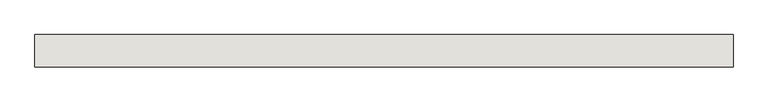
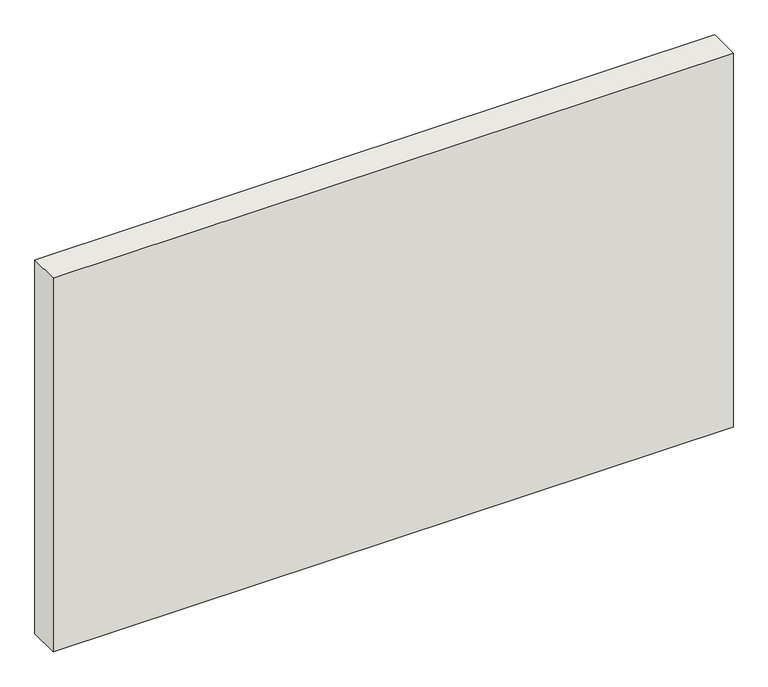
"""IFC4 building model written with IfcOpenShell, lengths in millimetres: wall geometry, Holzwand."""

from ifc_helpers import new_model, si_unit, origin, origin_with_axes, place, context, project, spatial, polyline, outline, extrude, source, transform, mapped, element, save


def wall_2eec8b8f(model_context):
    return source(origin(), model_context, "Body", "SweptSolid", [
        extrude(outline(polyline([(4297.8619019, 200.0), (4297.8619019, 0.0), (0.0, 0.0), (0.0, 200.0), (4297.8619019, 200.0)])), origin_with_axes(), (0.0, 0.0, 1.0), 2500.0),
    ])


if __name__ == "__main__":
    model = new_model("IFC4")
    model_context = context("Model", 3, world=origin())
    ifc_project = project(units=[si_unit("LENGTHUNIT", "METRE", prefix="MILLI")], contexts=[model_context])
    site = spatial("IfcSite", under=ifc_project)
    building = spatial("IfcBuilding", under=site)
    placement = place(None, origin())
    wall_shape = wall_2eec8b8f(model_context)
    element("IfcWall", 1, ObjectType="Holzwand", at=placement, inside=building, context=model_context, shape_type="MappedRepresentation", body=[
        mapped(wall_shape, transform((0.0, 0.0, 0.0), x_axis=(1.0, 0.0, 0.0), y_axis=(0.0, 1.0, 0.0), z_axis=(0.0, 0.0, 1.0))),
    ])
    save(model, "model.ifc")

# Revit data of these elements
# Element 1 (IfcWall, "Holzwand")
#   Materials on its faces: "holzschalung"
# Materials
#   "holzschalung": class "Unassigned", colour RGB 128 128 128, transparency 0
